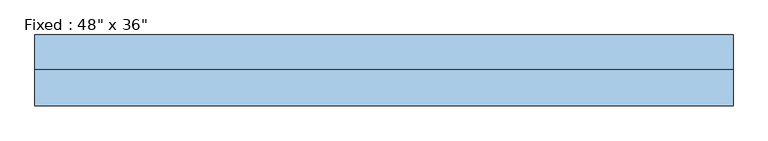
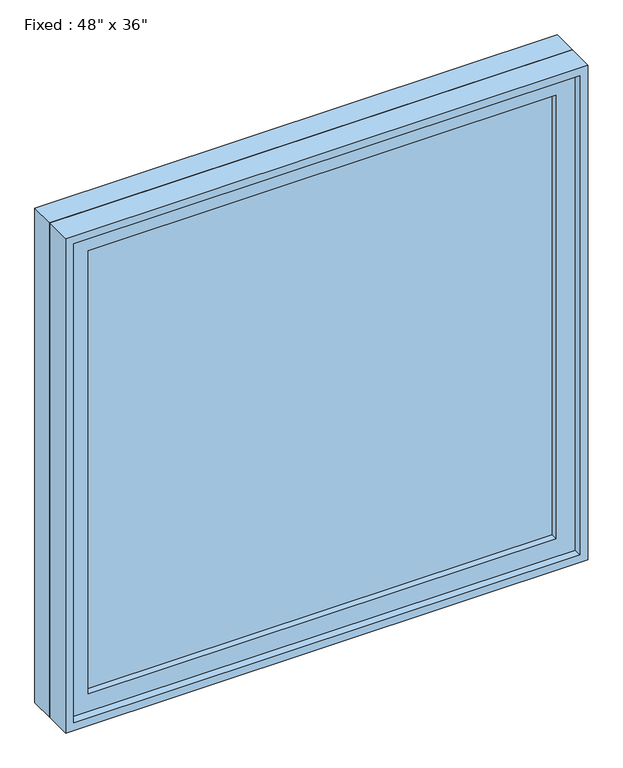
"""IFC4 building model written with IfcOpenShell, lengths in millimetres: window geometry."""

import ifcopenshell
import ifcopenshell.guid

model = None  # the IFC model being written
_history = None  # IfcOwnerHistory: only IFC2X3 demands one
_inside = {}  # id of a spatial element -> (the spatial element, [elements in it])
_under = {}  # id of a project, library or spatial element -> (it, [spatial elements below it])
_declared = {}  # id of a project -> (the project, [libraries it declares])
_typed = {}  # id of a type object -> (the type object, [elements of that type])
_made_of = {}  # id of a material, layer set ... -> (it, [elements and type objects made of it])


def new_model(schema):
    """Start an empty IFC model of exactly this schema.

    Asked for "IFC4X3", IfcOpenShell would pick the latest addendum, in which some entities
    have other attributes; the version numbers below select the first issue.
    IFC2X3 requires an IfcOwnerHistory on every rooted entity: one is made here for all.
    """
    global model, _history
    if schema == "IFC4X3":
        model = ifcopenshell.file(schema_version=(4, 3, 0, 0))
    else:
        model = ifcopenshell.file(schema=schema)
    _inside.clear()
    _under.clear()
    _declared.clear()
    _typed.clear()
    _made_of.clear()
    _history = None
    if model.schema == "IFC2X3":
        org = make("IfcOrganization", Name="unknown")
        user = make(
            "IfcPersonAndOrganization",
            ThePerson=make("IfcPerson", FamilyName="unknown"),
            TheOrganization=org,
        )
        app = make(
            "IfcApplication",
            ApplicationDeveloper=org,
            Version="unknown",
            ApplicationFullName="unknown",
            ApplicationIdentifier="unknown",
        )
        _history = make(
            "IfcOwnerHistory",
            OwningUser=user,
            OwningApplication=app,
            ChangeAction="ADDED",
            CreationDate=0,
        )
    return model


def make(cls, **values):
    """One entity of the class cls with the attributes given. An attribute that is None is left unset."""
    return model.create_entity(
        cls, **{name: value for name, value in values.items() if value is not None}
    )


def rooted(cls, **values):
    """An entity with a GlobalId (a new one), such as an element, a storey or a relation."""
    return make(cls, GlobalId=ifcopenshell.guid.new(), OwnerHistory=_history, **values)


def si_unit(unit_type, name, prefix=None):
    """IfcSIUnit, for example si_unit("LENGTHUNIT", "METRE", prefix="MILLI")."""
    return make("IfcSIUnit", UnitType=unit_type, Prefix=prefix, Name=name)


def assignment(units):
    """IfcUnitAssignment: the units of a project."""
    return None if units is None else make("IfcUnitAssignment", Units=units)


def point(xyz):
    """IfcCartesianPoint."""
    return None if xyz is None else make("IfcCartesianPoint", Coordinates=xyz)


def direction(xyz):
    """IfcDirection."""
    return None if xyz is None else make("IfcDirection", DirectionRatios=xyz)


def frame(location, z_axis=None, x_axis=None):
    """IfcAxis2Placement3D, a coordinate frame: its origin and axes. An axis left out is left unset."""
    return make(
        "IfcAxis2Placement3D",
        Location=point(location),
        Axis=direction(z_axis),
        RefDirection=direction(x_axis),
    )


def origin():
    """The frame at (0, 0, 0) with its axes left unset."""
    return frame((0.0, 0.0, 0.0))


def place(relative_to, where):
    """IfcLocalPlacement: puts the frame where relative to a parent placement (None: the world)."""
    return make(
        "IfcLocalPlacement", PlacementRelTo=relative_to, RelativePlacement=where
    )


def context(
    kind, dimensions, precision=None, world=None, true_north=None, identifier=None
):
    """IfcGeometricRepresentationContext, for example the 3D "Model" context."""
    return make(
        "IfcGeometricRepresentationContext",
        ContextIdentifier=identifier,
        ContextType=kind,
        CoordinateSpaceDimension=dimensions,
        Precision=precision,
        WorldCoordinateSystem=world,
        TrueNorth=true_north,
    )


def project(units=None, contexts=None):
    """IfcProject with its units and contexts."""
    return rooted(
        "IfcProject",
        Name="project",
        RepresentationContexts=contexts,
        UnitsInContext=assignment(units),
    )


def spatial(cls, under=None, at=None, **own):
    """A site, building, storey or space (cls), placed at a placement, below another one or the project."""
    s = rooted(cls, ObjectPlacement=at, **own)
    if under is not None:
        _under.setdefault(under.id(), (under, []))[1].append(s)
    return s


def polyline(points):
    """IfcPolyline through the points."""
    return make("IfcPolyline", Points=[point(p) for p in points])


def outline(outer, holes=None, kind="AREA"):
    """IfcArbitraryClosedProfileDef: a profile drawn as a closed curve; with holes, ...WithVoids."""
    if holes is None:
        return make("IfcArbitraryClosedProfileDef", ProfileType=kind, OuterCurve=outer)
    return make(
        "IfcArbitraryProfileDefWithVoids",
        ProfileType=kind,
        OuterCurve=outer,
        InnerCurves=holes,
    )


def extrude(swept, where, along, depth):
    """IfcExtrudedAreaSolid: the profile swept, set in the frame where, extruded along a direction by depth."""
    return make(
        "IfcExtrudedAreaSolid",
        SweptArea=swept,
        Position=where,
        ExtrudedDirection=direction(along),
        Depth=depth,
    )


def shape(context_of_items, identifier, shape_type, items):
    """IfcShapeRepresentation: the items that make up one representation, for example the "Body"."""
    return make(
        "IfcShapeRepresentation",
        ContextOfItems=context_of_items,
        RepresentationIdentifier=identifier,
        RepresentationType=shape_type,
        Items=items,
    )


def source(mapping_origin, context_of_items, identifier, shape_type, items):
    """IfcRepresentationMap: a shape defined once, which mapped items show again and again."""
    return make(
        "IfcRepresentationMap",
        MappingOrigin=mapping_origin,
        MappedRepresentation=shape(context_of_items, identifier, shape_type, items),
    )


def transform(
    local_origin,
    x_axis=None,
    y_axis=None,
    z_axis=None,
    scale=None,
    scale2=None,
    scale3=None,
    uniform=True,
):
    """IfcCartesianTransformationOperator3D, or its non-uniform kind. x_axis, y_axis, z_axis: its Axis1, 2, 3."""
    if uniform:
        return make(
            "IfcCartesianTransformationOperator3D",
            Axis1=direction(x_axis),
            Axis2=direction(y_axis),
            LocalOrigin=point(local_origin),
            Scale=scale,
            Axis3=direction(z_axis),
        )
    return make(
        "IfcCartesianTransformationOperator3DnonUniform",
        Axis1=direction(x_axis),
        Axis2=direction(y_axis),
        LocalOrigin=point(local_origin),
        Scale=scale,
        Axis3=direction(z_axis),
        Scale2=scale2,
        Scale3=scale3,
    )


def mapped(mapping_source, mapping_target):
    """IfcMappedItem: shows the shape of a source again, moved by a transform."""
    return make(
        "IfcMappedItem", MappingSource=mapping_source, MappingTarget=mapping_target
    )


def made_of(thing, what):
    """Note that an element or type object is made of a material, layer set ...; save() writes the relation."""
    if what is not None:
        _made_of.setdefault(what.id(), (what, []))[1].append(thing)
    return thing


def element(
    cls,
    number,
    at=None,
    inside=None,
    cuts=None,
    type_object=None,
    material=None,
    context=None,
    identifier="Body",
    shape_type=None,
    held_by="IfcProductDefinitionShape",
    body=None,
    shapes=None,
    **own,
):
    """One element of the class cls, such as IfcWall. Its Tag is "e" and its number.

    at: its placement. inside: the storey or other place that contains it. cuts: it is an
    opening in that element (IfcRelVoidsElement). A single representation is given by context,
    identifier, shape_type and body (its items); several are given by shapes. held_by: the class
    of the entity that holds the representations. save() writes the other relations.
    """
    e = rooted(cls, Tag="e%d" % number, ObjectPlacement=at, **own)
    if body is not None:
        shapes = [shape(context, identifier, shape_type, body)]
    if shapes is not None:
        e.Representation = make(held_by, Representations=shapes)
    if inside is not None:
        _inside.setdefault(inside.id(), (inside, []))[1].append(e)
    if cuts is not None:
        rooted(
            "IfcRelVoidsElement", RelatingBuildingElement=cuts, RelatedOpeningElement=e
        )
    if type_object is not None:
        _typed.setdefault(type_object.id(), (type_object, []))[1].append(e)
    return made_of(e, material)


def aggregate(whole, parts):
    """IfcRelAggregates: a whole, such as a stair, and the parts it consists of."""
    return rooted("IfcRelAggregates", RelatingObject=whole, RelatedObjects=parts)


def save(model, path):
    """Write the relations noted so far, then the file.

    IfcRelAggregates (storeys below a building ...), IfcRelContainedInSpatialStructure (elements
    in a storey), IfcRelDefinesByType, IfcRelAssociatesMaterial and IfcRelDeclares: one each for
    every whole, place, type object, material and project.
    """
    for whole, parts in _under.values():
        aggregate(whole, parts)
    for where, things in _inside.values():
        rooted(
            "IfcRelContainedInSpatialStructure",
            RelatedElements=things,
            RelatingStructure=where,
        )
    for kind, things in _typed.values():
        rooted("IfcRelDefinesByType", RelatedObjects=things, RelatingType=kind)
    for what, things in _made_of.values():
        rooted("IfcRelAssociatesMaterial", RelatedObjects=things, RelatingMaterial=what)
    for by, libraries in _declared.values():
        rooted("IfcRelDeclares", RelatingContext=by, RelatedDefinitions=libraries)
    model.write(path)


def window_33a7190b(model_context):
    return source(origin(), model_context, "Body", "SweptSolid", [
        extrude(outline(polyline([(508.0, -14.2875), (508.0, -26.9875), (-584.2, -26.9875), (-584.2, -14.2875), (508.0, -14.2875)])), frame((0.0, 0.0, 977.9), z_axis=(0.0, 0.0, 1.0), x_axis=(1.0, 0.0, 0.0)), (0.0, 0.0, 1.0), 1092.2),
        extrude(outline(polyline([(2114.55, -628.65), (933.45, -628.65), (933.45, 552.45), (2114.55, 552.45), (2114.55, -628.65)]), holes=[polyline([(2070.1, -584.2), (2070.1, 508.0), (977.9, 508.0), (977.9, -584.2), (2070.1, -584.2)])]), frame((0.0, -42.8625, 0.0), z_axis=(0.0, 1.0, 0.0), x_axis=(0.0, 0.0, 1.0)), (0.0, 0.0, 1.0), 44.45),
        extrude(outline(polyline([(2133.6, -647.7), (914.4, -647.7), (914.4, 571.5), (2133.6, 571.5), (2133.6, -647.7)]), holes=[polyline([(2101.85, -615.95), (2101.85, 539.75), (946.15, 539.75), (946.15, -615.95), (2101.85, -615.95)])]), frame((0.0, 1.5875, 0.0), z_axis=(0.0, 1.0, 0.0), x_axis=(0.0, 0.0, 1.0)), (0.0, 0.0, 1.0), 60.325),
        extrude(outline(polyline([(2133.6, 571.5), (2133.6, -647.7), (914.4, -647.7), (914.4, 571.5), (2133.6, 571.5)]), holes=[polyline([(2114.55, 552.45), (933.45, 552.45), (933.45, -628.65), (2114.55, -628.65), (2114.55, 552.45)])]), frame((0.0, -61.9125, 0.0), z_axis=(0.0, 1.0, 0.0), x_axis=(0.0, 0.0, 1.0)), (0.0, 0.0, 1.0), 63.5),
    ])


if __name__ == "__main__":
    model = new_model("IFC4")
    model_context = context("Model", 3, world=origin())
    ifc_project = project(units=[si_unit("LENGTHUNIT", "METRE", prefix="MILLI")], contexts=[model_context])
    site = spatial("IfcSite", under=ifc_project)
    building = spatial("IfcBuilding", under=site)
    placement = place(None, origin())
    window_shape = window_33a7190b(model_context)
    element("IfcWindow", 1, ObjectType="Fixed : 48\" x 36\"", at=placement, inside=building, context=model_context, shape_type="MappedRepresentation", body=[
        mapped(window_shape, transform((0.0, 0.0, 0.0), x_axis=(1.0, 0.0, 0.0), y_axis=(0.0, 1.0, 0.0), z_axis=(0.0, 0.0, 1.0))),
    ])
    save(model, "model.ifc")

# Revit data of these elements
# Type "Fixed : 48\" x 36\""
#   Type Mark = "10"
#   Assembly Code = "B2020100"
#   Height = 4' - 0"
#   Default Sill Height = 3' - 0"
#   Width = 4' - 0"
#   Window Inset = 0' - 0 3/4"
#   Glass Pane Material = Glass
#   Sash Material = Sash
#   Wall Closure = (empty or 0)
# Element 1 (IfcWindow, "Fixed : 48\" x 36\"")
#   Materials on its faces: "Sash", "Glass"
# Materials
#   "Glass": class "Glass", colour RGB 0 128 192, transparency 0.75
#   "Sash": class "Wood", colour RGB 224 178 126, transparency 0
